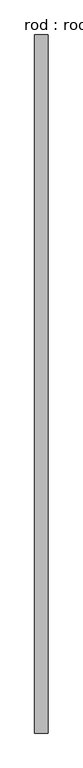
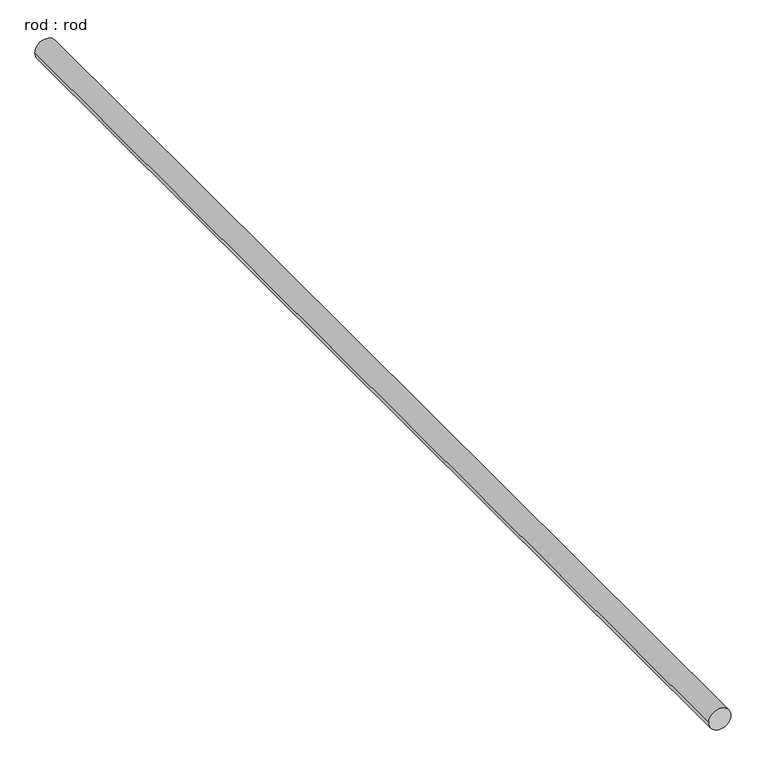
"""IFC4 building model written with IfcOpenShell, lengths in millimetres: proxy geometry, rod : rod."""

from ifc_helpers import new_model, si_unit, point, frame, frame_2d, origin, place, context, project, spatial, circle_curve, trimmed, segment, composite_curve, outline, extrude, source, transform, mapped, element, save


def rod_rod_10021e49(model_context):
    return source(origin(), model_context, "Body", "SweptSolid", [
        extrude(outline(composite_curve([segment(trimmed(circle_curve(frame_2d((0.0108462, 0.0)), 200.0), [point((0.0108462, 200.0))], [point((0.0108462, -200.0))], False, "CARTESIAN"), True, "CONTINUOUS"), segment(trimmed(circle_curve(frame_2d((0.0108462, 0.0)), 200.0), [point((0.0108462, -200.0))], [point((0.0108462, 200.0))], False, "CARTESIAN"), True, "CONTINUOUS")], self_intersect=False)), frame((0.0, -6407.2713847, 0.0), z_axis=(0.0, 1.0, 0.0), x_axis=(0.0, 0.0, 1.0)), (0.0, 0.0, 1.0), 21000.0),
    ])


if __name__ == "__main__":
    model = new_model("IFC4")
    model_context = context("Model", 3, world=origin())
    ifc_project = project(units=[si_unit("LENGTHUNIT", "METRE", prefix="MILLI")], contexts=[model_context])
    site = spatial("IfcSite", under=ifc_project)
    building = spatial("IfcBuilding", under=site)
    placement = place(None, origin())
    rod_rod_shape = rod_rod_10021e49(model_context)
    element("IfcBuildingElementProxy", 1, Name="rod : rod", ObjectType="rod : rod", at=placement, inside=building, context=model_context, shape_type="MappedRepresentation", body=[
        mapped(rod_rod_shape, transform((0.0, 0.0, 0.0), x_axis=(1.0, 0.0, 0.0), y_axis=(0.0, 1.0, 0.0), z_axis=(0.0, 0.0, 1.0))),
    ])
    save(model, "model.ifc")

# Revit data of these elements
# Type "rod : rod"
#   Default Elevation = 0
